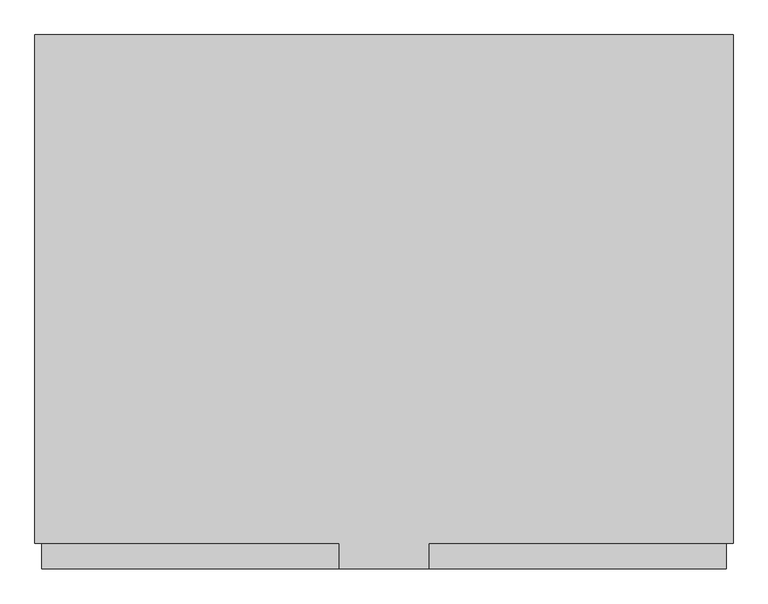
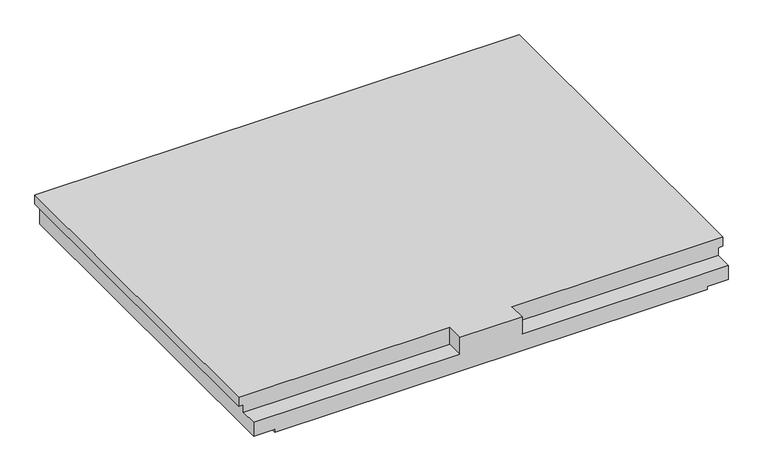
"""IFC4 building model written with IfcOpenShell, lengths in millimetres: stair geometry, NLRS_24_GM_UN_rechthoekig bordes prefab-AV_gen_rsf : prefab bordes_gen__2300x3005."""

from ifc_helpers import new_model, si_unit, origin, place, context, project, spatial, faceted_brep, source, transform, mapped, element, save


def stair_8b033359(model_context):
    return source(origin(), model_context, "Body", "Brep", [
        faceted_brep([(1502.5, -2190.0, 0.0), (1502.5, -2190.0, -60.0), (1502.5, 0.0, -60.0), (1502.5, 0.0, 0.0), (192.5, -2300.0, -110.0), (1472.5, -2300.0, -110.0), (1472.5, -2190.0, -110.0), (192.5, -2190.0, -110.0), (192.5, -2190.0, 0.0), (1472.5, -2190.0, -60.0), (192.5, -2300.0, 0.0), (-192.5, -2300.0, 0.0), (-192.5, -2190.0, 0.0), (-192.5, -2190.0, -110.0), (-192.5, -2300.0, -110.0), (-1502.5, 0.0, 0.0), (-1502.5, 0.0, -60.0), (-1502.5, -2190.0, -60.0), (-1502.5, -2190.0, 0.0), (-1472.5, -2300.0, -110.0), (-1472.5, -2300.0, -200.0), (-1342.5, -2300.0, -200.0), (-1342.5, -2300.0, -220.0), (1342.5, -2300.0, -220.0), (1342.5, -2300.0, -200.0), (1472.5, -2300.0, -200.0), (-1472.5, -2190.0, -110.0), (-1472.5, -2190.0, -60.0), (1472.5, 0.0, -60.0), (1472.5, 0.0, -200.0), (1342.5, 0.0, -200.0), (1342.5, 0.0, -220.0), (-1342.5, 0.0, -220.0), (-1342.5, 0.0, -200.0), (-1472.5, 0.0, -200.0), (-1472.5, 0.0, -60.0)], [[[0, 1, 2, 3]], [[4, 5, 6, 7]], [[8, 7, 6, 9, 1, 0]], [[10, 4, 7, 8]], [[11, 12, 13, 14]], [[15, 16, 17, 18]], [[19, 20, 21, 22, 23, 24, 25, 5, 4, 10, 11, 14]], [[14, 13, 26, 19]], [[18, 17, 27, 26, 13, 12]], [[18, 12, 11, 10, 8, 0, 3, 15]], [[15, 3, 2, 28, 29, 30, 31, 32, 33, 34, 35, 16]], [[32, 31, 23, 22]], [[27, 17, 16, 35]], [[20, 19, 26, 27, 35, 34]], [[34, 33, 21, 20]], [[33, 32, 22, 21]], [[28, 2, 1, 9]], [[29, 28, 9, 6, 5, 25]], [[25, 24, 30, 29]], [[24, 23, 31, 30]]]),
    ])


if __name__ == "__main__":
    model = new_model("IFC4")
    model_context = context("Model", 3, world=origin())
    ifc_project = project(units=[si_unit("LENGTHUNIT", "METRE", prefix="MILLI")], contexts=[model_context])
    site = spatial("IfcSite", under=ifc_project)
    building = spatial("IfcBuilding", under=site)
    placement = place(None, origin())
    stair_shape = stair_8b033359(model_context)
    element("IfcStair", 1, ObjectType="NLRS_24_GM_UN_rechthoekig bordes prefab-AV_gen_rsf : prefab bordes_gen__2300x3005", at=placement, inside=building, context=model_context, shape_type="MappedRepresentation", body=[
        mapped(stair_shape, transform((0.0, 0.0, 0.0), x_axis=(1.0, 0.0, 0.0), y_axis=(0.0, 1.0, 0.0), z_axis=(0.0, 0.0, 1.0))),
    ])
    save(model, "model.ifc")

# Revit data of these elements
# Type "NLRS_24_GM_UN_rechthoekig bordes prefab-AV_gen_rsf : prefab bordes_gen__2300x3005"
#   IfcExportAs = "IfcStair"
#   Type Comments = " "
#   Model = " "
#   Manufacturer = " "
#   Description = "rechthoekig bordes prefab\r\n1930x4395"
#   Assembly Code = "24.15"
#   Width = 3005 mm
#   Thickness = 220 mm
#   Perimeter = 10610 mm
#   NLRS_C_lengte_02 = 1310 mm
#   NLRS_C_lengte_01 = 1310 mm
#   NLRS_C_hoogte_02 = 110 mm
#   NLRS_C_hoogte_01 = 110 mm
#   NLRS_C_diepte_04 = 2300 mm
#   NLRS_C_diepte_03 = 2300 mm
#   NLRS_C_diepte_02 = 110 mm
#   NLRS_C_diepte_01 = 110 mm
#   Length = 2300 mm
#   Default Elevation = 1219.2 mm
#   Area = 6.9115 m²
#   NLRS_C_materiaal = NLRS_f2_beton prefab_gen_rsf
#   Keynote = ""
# Element 1 (IfcStair, "NLRS_24_GM_UN_rechthoekig bordes prefab-AV_gen_rsf : prefab bordes_gen__2300x3005")
#   Materials on its faces: "NLRS_f2_beton prefab_gen_rsf"
# Materials
#   "NLRS_f2_beton prefab_gen_rsf": class "F - Niet gebakken kunststeen", colour RGB 129 133 118, transparency 0, Keynote = "f2", Manufacturer = "Revit Standards Foundation", URL = "www.revitstandards.org", Description = "beton prefab", Cost = 0
